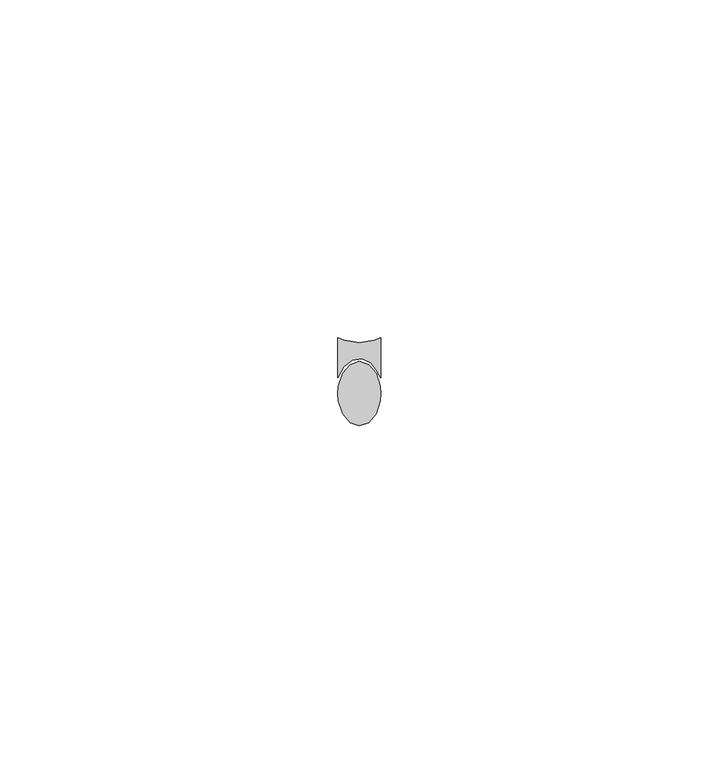
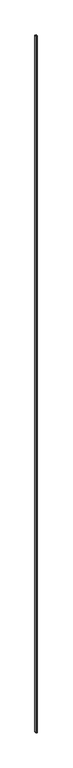
"""IFC4 building model written with IfcOpenShell, lengths in millimetres: proxy geometry, Generic Models 11:Generic Models 1:306267:Generic Models 1:306267 : Generic Models 11:Generic Models 1:306267:300405:Generic Models 1:306267:Generic Models 1:306267 : Generic Models 11:Generic Models 1:306267:300405 : Generic Models 11:Generic Models 1:306267:Generic Models 1:306267 : Generic Models 11:Generic Models 1:306267:300405:28 : Generic Models 11:Generic Models 1:306267:Generic Models 1:306267 : Generic Models 11:Generic Models 1:306267:300405:Generic Models 1:306267:Generic Models 1:306267 : Generic Models 11:Generic Models 1:306267:300405 : Generic Models 11:Generic Models 1:306267:Generic Models 1:306267 : Generic Models 11:Generic Models 1:306267:300405:300182."""

from ifc_helpers import new_model, si_unit, frame, origin, place, context, project, spatial, polyline, outline, extrude, source, transform, mapped, element, save


def generic_models_a726f077(model_context):
    return source(origin(), model_context, "Body", "SweptSolid", [
        extrude(outline(polyline([(593732.7024872, -579004.2437927), (593734.9117239, -579004.5574788), (593737.1209607, -579004.2437927), (593738.0867239, -579003.8663841), (593738.0867239, -579009.7344762), (593737.3327483, -579008.4767657), (593736.6169209, -579007.5646201), (593735.2666732, -579006.9642666), (593733.8608969, -579007.1670545), (593732.6195128, -579008.1412595), (593731.7367239, -579009.7344762), (593731.7367239, -579003.8663841), (593732.7024872, -579004.2437927)])), frame((0.0, 0.0, 31.75), z_axis=(0.0, 0.0, 1.0), x_axis=(1.0, 0.0, 0.0)), (0.0, 0.0, 1.0), 3670.3),
        extrude(outline(polyline([(593736.2893048, -579007.8072396), (593737.3940389, -579009.1287336), (593738.0071201, -579011.0383478), (593738.0867239, -579012.0981038), (593738.0071201, -579013.1578597), (593737.3940389, -579015.067474), (593736.2893048, -579016.388968), (593734.9117239, -579016.8606038), (593733.5341431, -579016.388968), (593732.429409, -579015.067474), (593731.8163278, -579013.1578597), (593731.7367239, -579012.0981038), (593731.8163278, -579011.0383478), (593732.429409, -579009.1287336), (593733.5341431, -579007.8072396), (593734.9117239, -579007.3356038), (593736.2893048, -579007.8072396)])), frame((0.0, 0.0, 31.75), z_axis=(0.0, 0.0, 1.0), x_axis=(1.0, 0.0, 0.0)), (0.0, 0.0, 1.0), 3670.3),
    ])


if __name__ == "__main__":
    model = new_model("IFC4")
    model_context = context("Model", 3, world=origin())
    ifc_project = project(units=[si_unit("LENGTHUNIT", "METRE", prefix="MILLI")], contexts=[model_context])
    site = spatial("IfcSite", under=ifc_project)
    building = spatial("IfcBuilding", under=site)
    placement = place(None, origin())
    generic_models_shape = generic_models_a726f077(model_context)
    element("IfcBuildingElementProxy", 1, Name="Generic Models 11:Generic Models 1:306267:Generic Models 1:306267 : Generic Models 11:Generic Models 1:306267:300405:Generic Models 1:306267:Generic Models 1:306267 : Generic Models 11:Generic Models 1:306267:300405 : Generic Models 11:Generic Models 1:306267:Generic Models 1:306267 : Generic Models 11:Generic Models 1:306267:300405:28 : Generic Models 11:Generic Models 1:306267:Generic Models 1:306267 : Generic Models 11:Generic Models 1:306267:300405:Generic Models 1:306267:Generic Models 1:306267 : Generic Models 11:Generic Models 1:306267:300405 : Generic Models 11:Generic Models 1:306267:Generic Models 1:306267 : Generic Models 11:Generic Models 1:306267:300405:300182", ObjectType="Generic Models 11:Generic Models 1:306267:Generic Models 1:306267 : Generic Models 11:Generic Models 1:306267:300405:Generic Models 1:306267:Generic Models 1:306267 : Generic Models 11:Generic Models 1:306267:300405 : Generic Models 11:Generic Models 1:306267:Generic Models 1:306267 : Generic Models 11:Generic Models 1:306267:300405:28 : Generic Models 11:Generic Models 1:306267:Generic Models 1:306267 : Generic Models 11:Generic Models 1:306267:300405:Generic Models 1:306267:Generic Models 1:306267 : Generic Models 11:Generic Models 1:306267:300405 : Generic Models 11:Generic Models 1:306267:Generic Models 1:306267 : Generic Models 11:Generic Models 1:306267:300405:300182", at=placement, inside=building, context=model_context, shape_type="MappedRepresentation", body=[
        mapped(generic_models_shape, transform((0.0, 0.0, 0.0), x_axis=(1.0, 0.0, 0.0), y_axis=(0.0, 1.0, 0.0), z_axis=(0.0, 0.0, 1.0))),
    ])
    save(model, "model.ifc")

# Revit data of these elements
# Type "Generic Models 11:Generic Models 1:306267:Generic Models 1:306267 : Generic Models 11:Generic Models 1:306267:300405:Generic Models 1:306267:Generic Models 1:306267 : Generic Models 11:Generic Models 1:306267:300405 : Generic Models 11:Generic Models 1:306267:Generic Models 1:306267 : Generic Models 11:Generic Models 1:306267:300405:28 : Generic Models 11:Generic Models 1:306267:Generic Models 1:306267 : Generic Models 11:Generic Models 1:306267:300405:Generic Models 1:306267:Generic Models 1:306267 : Generic Models 11:Generic Models 1:306267:300405 : Generic Models 11:Generic Models 1:306267:Generic Models 1:306267 : Generic Models 11:Generic Models 1:306267:300405:300182"
#   NameOverride = "Generic Models 11:Generic Models 1:306267:Generic Models 1:306267 : Generic Models 11:Generic Models 1:306267:300405:Generic Models 1:306267:Generic Models 1:306267 : Generic Models 11:Generic Models 1:306267:300405 : Generic Models 11:Generic Models 1:306267:Generic Models 1:306267 : Generic Models 11:Generic Models 1:306267:300405:300182"
#   ObjectTypeOverride = "Generic Models 1:306267:Generic Models 1:306267 : Generic Models 11:Generic Models 1:306267:300405 : Generic Models 11:Generic Models 1:306267:Generic Models 1:306267 : Generic Models 11:Generic Models 1:306267:300405"
#   Reference = "Generic Models 1"
#   Tag = "300182"
# Element 1 (IfcBuildingElementProxy, "Generic Models 11:Generic Models 1:306267:Generic Models 1:306267 : Generic Models 11:Generic Models 1:306267:300405:Generic Models 1:306267:Generic Models 1:306267 : Generic Models 11:Generic Models 1:306267:300405 : Generic Models 11:Generic Models 1:306267:Generic Models 1:306267 : Generic Models 11:Generic Models 1:306267:300405:28 : Generic Models 11:Generic Models 1:306267:Generic Models 1:306267 : Generic Models 11:Generic Models 1:306267:300405:Generic Models 1:306267:Generic Models 1:306267 : Generic Models 11:Generic Models 1:306267:300405 : Generic Models 11:Generic Models 1:306267:Generic Models 1:306267 : Generic Models 11:Generic Models 1:306267:300405:300182")
#   Materials on its faces: "SEALANT & BACKER ROD, IF NECESSARY"
# Materials
#   "SEALANT & BACKER ROD, IF NECESSARY": class "Unassigned", colour RGB 120 120 120, transparency 0, Cost = 0
